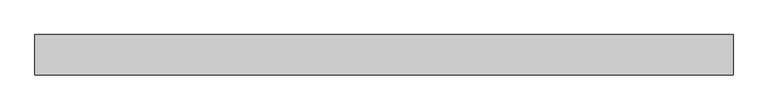
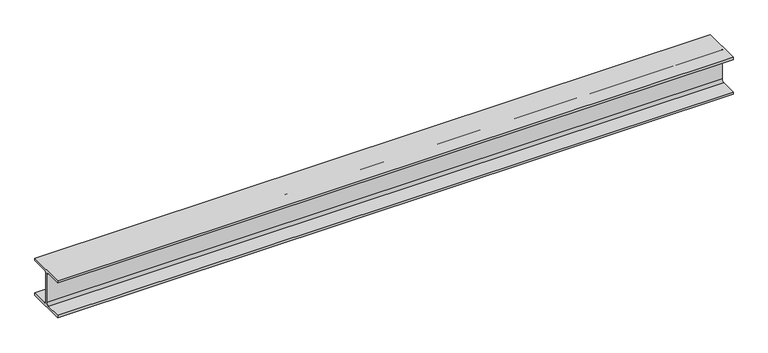
"""IFC4 building model written with IfcOpenShell, lengths in millimetres: beam geometry, 0912_Steel Framing_H-KSD3502 : H_SB_ASB_H-200x200x8x12."""

from ifc_helpers import new_model, si_unit, point, frame, frame_2d, origin, place, context, project, spatial, polyline, circle_curve, trimmed, segment, composite_curve, outline, extrude, source, transform, mapped, element, save


def beam_0eb71ca4(model_context):
    return source(origin(), model_context, "Body", "SweptSolid", [
        extrude(outline(composite_curve([segment(polyline([(100.0, -88.0), (100.0, -100.0), (-100.0, -100.0), (-100.0, -88.0), (-17.0, -88.0)]), True, "CONTINUOUS"), segment(trimmed(circle_curve(frame_2d((-17.0, -75.0)), 13.0), [point((-17.0, -88.0))], [point((-4.0, -75.0))], True, "CARTESIAN"), True, "CONTINUOUS"), segment(polyline([(-4.0, -75.0), (-4.0, 75.0)]), True, "CONTINUOUS"), segment(trimmed(circle_curve(frame_2d((-17.0, 75.0)), 13.0), [point((-4.0, 75.0))], [point((-17.0, 88.0))], True, "CARTESIAN"), True, "CONTINUOUS"), segment(polyline([(-17.0, 88.0), (-100.0, 88.0), (-100.0, 100.0), (100.0, 100.0), (100.0, 88.0), (17.0, 88.0)]), True, "CONTINUOUS"), segment(trimmed(circle_curve(frame_2d((17.0, 75.0)), 13.0), [point((17.0, 88.0))], [point((4.0, 75.0))], True, "CARTESIAN"), True, "CONTINUOUS"), segment(polyline([(4.0, 75.0), (4.0, -75.0)]), True, "CONTINUOUS"), segment(trimmed(circle_curve(frame_2d((17.0, -75.0)), 13.0), [point((4.0, -75.0))], [point((17.0, -88.0))], True, "CARTESIAN"), True, "CONTINUOUS"), segment(polyline([(17.0, -88.0), (100.0, -88.0)]), True, "CONTINUOUS")], self_intersect=False)), frame((-1683.7594404, 0.0, 0.0), z_axis=(1.0, 0.0, 0.0), x_axis=(0.0, 1.0, 0.0)), (0.0, 0.0, 1.0), 3450.380526),
    ])


if __name__ == "__main__":
    model = new_model("IFC4")
    model_context = context("Model", 3, world=origin())
    ifc_project = project(units=[si_unit("LENGTHUNIT", "METRE", prefix="MILLI")], contexts=[model_context])
    site = spatial("IfcSite", under=ifc_project)
    building = spatial("IfcBuilding", under=site)
    placement = place(None, origin())
    beam_shape = beam_0eb71ca4(model_context)
    element("IfcBeam", 1, ObjectType="0912_Steel Framing_H-KSD3502 : H_SB_ASB_H-200x200x8x12", at=placement, inside=building, context=model_context, shape_type="MappedRepresentation", body=[
        mapped(beam_shape, transform((0.0, 0.0, 0.0), x_axis=(1.0, 0.0, 0.0), y_axis=(0.0, 1.0, 0.0), z_axis=(0.0, 0.0, 1.0))),
    ])
    save(model, "model.ifc")

# Revit data of these elements
# Type "0912_Steel Framing_H-KSD3502 : H_SB_ASB_H-200x200x8x12"
#   H_WM Code_1 = "S01AA002-00001 | Main Steel Structure Fabrication Work | Shelter/Building | Medium Steel - Standard (90KG/M>Weight≥30KG/M) | Material: (   )"
#   H_WM Code_2 = "S03AA028-00001 | Main Steel Structure Erection Work | Shelter/Building | Medium Steel (90KG/M>Weight≥30KG/M) | Material: (   )"
#   H_WM Code_3 = "S01AA010-00001 | Main Steel Structure Fabrication Work | Shelter/Building | Steel Painting/Coating | for Non-Fireproofed Steel Surface, Surface Preparation, Primer, Second & Final Coat | Material: (   )"
#   H_Q'ty Cal Type Tag = "SB-Q2"
#   Width = 20.0 cm
#   Web Thickness = 0.8 cm
#   Web Fillet = 1.3 cm
#   Warping Constant = 141000.0 cm⁶
#   W = 0
#   Torsional Moment of Inertia = 26.2485 cm⁴
#   Section Area = 63.53 cm²
#   Plastic Modulus weak axis = 244.0 cm³
#   Plastic Modulus strong axis = 525.0 cm³
#   Perimeter = 1.16 m²/m
#   Nominal Weight = 49.90 kgf/m
#   Moment of Inertia weak axis = 1600.00 cm⁴
#   Moment of Inertia strong axis = 4720.00 cm⁴
#   Height = 20.0 cm
#   Flange Thickness = 1.2 cm
#   Elastic Modulus weak axis = 160.0 cm³
#   Elastic Modulus strong axis = 472.0 cm³
#   Centroid Vertical = 10.0 cm
#   Centroid Horizontal = 10.0 cm
#   Ix = 47200000
#   Length [instance default] = 1.5240 m
#   Zx = 525000
#   b = 0.2000 m
#   h = 0.2000 m
#   r = 0.0130 m
#   s = 0.0080 m
#   t = 0.0120 m
#   A = 0.006353 m²
#   Structural Material [instance default] = Steel, 45-345
#   Assembly Code = ""
# Element 1 (IfcBeam, "0912_Steel Framing_H-KSD3502 : H_SB_ASB_H-200x200x8x12")
#   Structural Material = none
# Materials
#   "Steel, 45-345": class "Metal", colour RGB 189 187 185, transparency 0, Description = "Steel 345 MPa", Cost = 0
